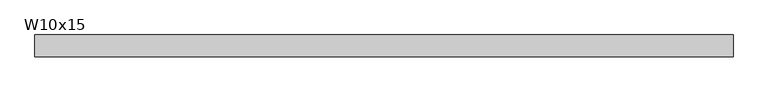
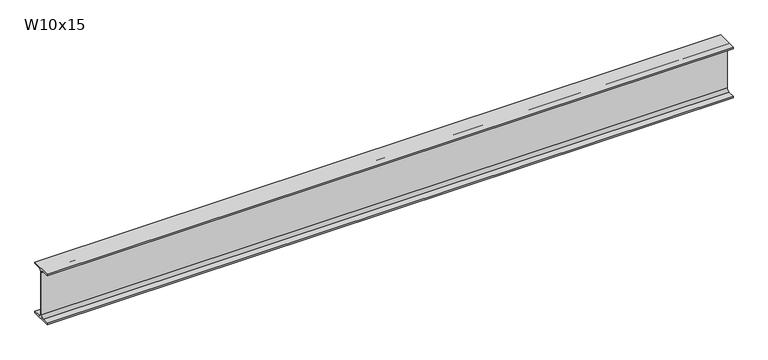
"""IFC4 building model written with IfcOpenShell, lengths in millimetres: beam geometry, RME W-Wide Flange : W10x15."""

import ifcopenshell
import ifcopenshell.guid

model = None  # the IFC model being written
_history = None  # IfcOwnerHistory: only IFC2X3 demands one
_inside = {}  # id of a spatial element -> (the spatial element, [elements in it])
_under = {}  # id of a project, library or spatial element -> (it, [spatial elements below it])
_declared = {}  # id of a project -> (the project, [libraries it declares])
_typed = {}  # id of a type object -> (the type object, [elements of that type])
_made_of = {}  # id of a material, layer set ... -> (it, [elements and type objects made of it])


def new_model(schema):
    """Start an empty IFC model of exactly this schema.

    Asked for "IFC4X3", IfcOpenShell would pick the latest addendum, in which some entities
    have other attributes; the version numbers below select the first issue.
    IFC2X3 requires an IfcOwnerHistory on every rooted entity: one is made here for all.
    """
    global model, _history
    if schema == "IFC4X3":
        model = ifcopenshell.file(schema_version=(4, 3, 0, 0))
    else:
        model = ifcopenshell.file(schema=schema)
    _inside.clear()
    _under.clear()
    _declared.clear()
    _typed.clear()
    _made_of.clear()
    _history = None
    if model.schema == "IFC2X3":
        org = make("IfcOrganization", Name="unknown")
        user = make(
            "IfcPersonAndOrganization",
            ThePerson=make("IfcPerson", FamilyName="unknown"),
            TheOrganization=org,
        )
        app = make(
            "IfcApplication",
            ApplicationDeveloper=org,
            Version="unknown",
            ApplicationFullName="unknown",
            ApplicationIdentifier="unknown",
        )
        _history = make(
            "IfcOwnerHistory",
            OwningUser=user,
            OwningApplication=app,
            ChangeAction="ADDED",
            CreationDate=0,
        )
    return model


def make(cls, **values):
    """One entity of the class cls with the attributes given. An attribute that is None is left unset."""
    return model.create_entity(
        cls, **{name: value for name, value in values.items() if value is not None}
    )


def rooted(cls, **values):
    """An entity with a GlobalId (a new one), such as an element, a storey or a relation."""
    return make(cls, GlobalId=ifcopenshell.guid.new(), OwnerHistory=_history, **values)


def si_unit(unit_type, name, prefix=None):
    """IfcSIUnit, for example si_unit("LENGTHUNIT", "METRE", prefix="MILLI")."""
    return make("IfcSIUnit", UnitType=unit_type, Prefix=prefix, Name=name)


def assignment(units):
    """IfcUnitAssignment: the units of a project."""
    return None if units is None else make("IfcUnitAssignment", Units=units)


def point(xyz):
    """IfcCartesianPoint."""
    return None if xyz is None else make("IfcCartesianPoint", Coordinates=xyz)


def direction(xyz):
    """IfcDirection."""
    return None if xyz is None else make("IfcDirection", DirectionRatios=xyz)


def frame(location, z_axis=None, x_axis=None):
    """IfcAxis2Placement3D, a coordinate frame: its origin and axes. An axis left out is left unset."""
    return make(
        "IfcAxis2Placement3D",
        Location=point(location),
        Axis=direction(z_axis),
        RefDirection=direction(x_axis),
    )


def frame_2d(location, x_axis=None):
    """IfcAxis2Placement2D, a coordinate frame in the plane: its origin and x axis."""
    return make(
        "IfcAxis2Placement2D", Location=point(location), RefDirection=direction(x_axis)
    )


def origin():
    """The frame at (0, 0, 0) with its axes left unset."""
    return frame((0.0, 0.0, 0.0))


def place(relative_to, where):
    """IfcLocalPlacement: puts the frame where relative to a parent placement (None: the world)."""
    return make(
        "IfcLocalPlacement", PlacementRelTo=relative_to, RelativePlacement=where
    )


def context(
    kind, dimensions, precision=None, world=None, true_north=None, identifier=None
):
    """IfcGeometricRepresentationContext, for example the 3D "Model" context."""
    return make(
        "IfcGeometricRepresentationContext",
        ContextIdentifier=identifier,
        ContextType=kind,
        CoordinateSpaceDimension=dimensions,
        Precision=precision,
        WorldCoordinateSystem=world,
        TrueNorth=true_north,
    )


def project(units=None, contexts=None):
    """IfcProject with its units and contexts."""
    return rooted(
        "IfcProject",
        Name="project",
        RepresentationContexts=contexts,
        UnitsInContext=assignment(units),
    )


def spatial(cls, under=None, at=None, **own):
    """A site, building, storey or space (cls), placed at a placement, below another one or the project."""
    s = rooted(cls, ObjectPlacement=at, **own)
    if under is not None:
        _under.setdefault(under.id(), (under, []))[1].append(s)
    return s


def polyline(points):
    """IfcPolyline through the points."""
    return make("IfcPolyline", Points=[point(p) for p in points])


def circle_curve(where, radius):
    """IfcCircle in the frame where."""
    return make("IfcCircle", Position=where, Radius=radius)


def trimmed(basis, trim1, trim2, sense, master):
    """IfcTrimmedCurve: the piece of a basis curve between two trims."""
    return make(
        "IfcTrimmedCurve",
        BasisCurve=basis,
        Trim1=trim1,
        Trim2=trim2,
        SenseAgreement=sense,
        MasterRepresentation=master,
    )


def segment(curve, same_sense, transition):
    """IfcCompositeCurveSegment."""
    return make(
        "IfcCompositeCurveSegment",
        Transition=transition,
        SameSense=same_sense,
        ParentCurve=curve,
    )


def composite_curve(segments, self_intersect=None):
    """IfcCompositeCurve: segments joined end to end."""
    return make("IfcCompositeCurve", Segments=segments, SelfIntersect=self_intersect)


def outline(outer, holes=None, kind="AREA"):
    """IfcArbitraryClosedProfileDef: a profile drawn as a closed curve; with holes, ...WithVoids."""
    if holes is None:
        return make("IfcArbitraryClosedProfileDef", ProfileType=kind, OuterCurve=outer)
    return make(
        "IfcArbitraryProfileDefWithVoids",
        ProfileType=kind,
        OuterCurve=outer,
        InnerCurves=holes,
    )


def extrude(swept, where, along, depth):
    """IfcExtrudedAreaSolid: the profile swept, set in the frame where, extruded along a direction by depth."""
    return make(
        "IfcExtrudedAreaSolid",
        SweptArea=swept,
        Position=where,
        ExtrudedDirection=direction(along),
        Depth=depth,
    )


def shape(context_of_items, identifier, shape_type, items):
    """IfcShapeRepresentation: the items that make up one representation, for example the "Body"."""
    return make(
        "IfcShapeRepresentation",
        ContextOfItems=context_of_items,
        RepresentationIdentifier=identifier,
        RepresentationType=shape_type,
        Items=items,
    )


def source(mapping_origin, context_of_items, identifier, shape_type, items):
    """IfcRepresentationMap: a shape defined once, which mapped items show again and again."""
    return make(
        "IfcRepresentationMap",
        MappingOrigin=mapping_origin,
        MappedRepresentation=shape(context_of_items, identifier, shape_type, items),
    )


def transform(
    local_origin,
    x_axis=None,
    y_axis=None,
    z_axis=None,
    scale=None,
    scale2=None,
    scale3=None,
    uniform=True,
):
    """IfcCartesianTransformationOperator3D, or its non-uniform kind. x_axis, y_axis, z_axis: its Axis1, 2, 3."""
    if uniform:
        return make(
            "IfcCartesianTransformationOperator3D",
            Axis1=direction(x_axis),
            Axis2=direction(y_axis),
            LocalOrigin=point(local_origin),
            Scale=scale,
            Axis3=direction(z_axis),
        )
    return make(
        "IfcCartesianTransformationOperator3DnonUniform",
        Axis1=direction(x_axis),
        Axis2=direction(y_axis),
        LocalOrigin=point(local_origin),
        Scale=scale,
        Axis3=direction(z_axis),
        Scale2=scale2,
        Scale3=scale3,
    )


def mapped(mapping_source, mapping_target):
    """IfcMappedItem: shows the shape of a source again, moved by a transform."""
    return make(
        "IfcMappedItem", MappingSource=mapping_source, MappingTarget=mapping_target
    )


def made_of(thing, what):
    """Note that an element or type object is made of a material, layer set ...; save() writes the relation."""
    if what is not None:
        _made_of.setdefault(what.id(), (what, []))[1].append(thing)
    return thing


def element(
    cls,
    number,
    at=None,
    inside=None,
    cuts=None,
    type_object=None,
    material=None,
    context=None,
    identifier="Body",
    shape_type=None,
    held_by="IfcProductDefinitionShape",
    body=None,
    shapes=None,
    **own,
):
    """One element of the class cls, such as IfcWall. Its Tag is "e" and its number.

    at: its placement. inside: the storey or other place that contains it. cuts: it is an
    opening in that element (IfcRelVoidsElement). A single representation is given by context,
    identifier, shape_type and body (its items); several are given by shapes. held_by: the class
    of the entity that holds the representations. save() writes the other relations.
    """
    e = rooted(cls, Tag="e%d" % number, ObjectPlacement=at, **own)
    if body is not None:
        shapes = [shape(context, identifier, shape_type, body)]
    if shapes is not None:
        e.Representation = make(held_by, Representations=shapes)
    if inside is not None:
        _inside.setdefault(inside.id(), (inside, []))[1].append(e)
    if cuts is not None:
        rooted(
            "IfcRelVoidsElement", RelatingBuildingElement=cuts, RelatedOpeningElement=e
        )
    if type_object is not None:
        _typed.setdefault(type_object.id(), (type_object, []))[1].append(e)
    return made_of(e, material)


def aggregate(whole, parts):
    """IfcRelAggregates: a whole, such as a stair, and the parts it consists of."""
    return rooted("IfcRelAggregates", RelatingObject=whole, RelatedObjects=parts)


def save(model, path):
    """Write the relations noted so far, then the file.

    IfcRelAggregates (storeys below a building ...), IfcRelContainedInSpatialStructure (elements
    in a storey), IfcRelDefinesByType, IfcRelAssociatesMaterial and IfcRelDeclares: one each for
    every whole, place, type object, material and project.
    """
    for whole, parts in _under.values():
        aggregate(whole, parts)
    for where, things in _inside.values():
        rooted(
            "IfcRelContainedInSpatialStructure",
            RelatedElements=things,
            RelatingStructure=where,
        )
    for kind, things in _typed.values():
        rooted("IfcRelDefinesByType", RelatedObjects=things, RelatingType=kind)
    for what, things in _made_of.values():
        rooted("IfcRelAssociatesMaterial", RelatedObjects=things, RelatingMaterial=what)
    for by, libraries in _declared.values():
        rooted("IfcRelDeclares", RelatingContext=by, RelatedDefinitions=libraries)
    model.write(path)


def w10x15_dad78829(model_context):
    return source(origin(), model_context, "Body", "SweptSolid", [
        extrude(outline(composite_curve([segment(polyline([(50.8, -120.142), (50.8, -127.0), (-50.8, -127.0), (-50.8, -120.142), (-16.7005, -120.142)]), True, "CONTINUOUS"), segment(trimmed(circle_curve(frame_2d((-16.7005, -106.3625)), 13.7795), [point((-16.7005, -120.142))], [point((-2.921, -106.3625))], True, "CARTESIAN"), True, "CONTINUOUS"), segment(polyline([(-2.921, -106.3625), (-2.921, 106.3625)]), True, "CONTINUOUS"), segment(trimmed(circle_curve(frame_2d((-16.7005, 106.3625)), 13.7795), [point((-2.921, 106.3625))], [point((-16.7005, 120.142))], True, "CARTESIAN"), True, "CONTINUOUS"), segment(polyline([(-16.7005, 120.142), (-50.8, 120.142), (-50.8, 127.0), (50.8, 127.0), (50.8, 120.142), (16.7005, 120.142)]), True, "CONTINUOUS"), segment(trimmed(circle_curve(frame_2d((16.7005, 106.3625)), 13.7795), [point((16.7005, 120.142))], [point((2.921, 106.3625))], True, "CARTESIAN"), True, "CONTINUOUS"), segment(polyline([(2.921, 106.3625), (2.921, -106.3625)]), True, "CONTINUOUS"), segment(trimmed(circle_curve(frame_2d((16.7005, -106.3625)), 13.7795), [point((2.921, -106.3625))], [point((16.7005, -120.142))], True, "CARTESIAN"), True, "CONTINUOUS"), segment(polyline([(16.7005, -120.142), (50.8, -120.142)]), True, "CONTINUOUS")], self_intersect=False)), frame((-1630.5983978, 0.0, 0.0), z_axis=(1.0, 0.0, 0.0), x_axis=(0.0, 1.0, 0.0)), (0.0, 0.0, 1.0), 3261.1967956),
    ])


if __name__ == "__main__":
    model = new_model("IFC4")
    model_context = context("Model", 3, world=origin())
    ifc_project = project(units=[si_unit("LENGTHUNIT", "METRE", prefix="MILLI")], contexts=[model_context])
    site = spatial("IfcSite", under=ifc_project)
    building = spatial("IfcBuilding", under=site)
    placement = place(None, origin())
    w10x15_shape = w10x15_dad78829(model_context)
    element("IfcBeam", 1, ObjectType="RME W-Wide Flange : W10x15", at=placement, inside=building, context=model_context, shape_type="MappedRepresentation", body=[
        mapped(w10x15_shape, transform((0.0, 0.0, 0.0), x_axis=(1.0, 0.0, 0.0), y_axis=(0.0, 1.0, 0.0), z_axis=(0.0, 0.0, 1.0))),
    ])
    save(model, "model.ifc")

# Revit data of these elements
# Type "RME W-Wide Flange : W10x15"
#   WELD P [instance default] = ""
#   WELD LE [instance default] = ""
#   WELD D [instance default] = ""
#   TOP SECTION SIZE [instance default] = ""
#   TOP SECTION LENGTH [instance default] = ""
#   REMARKS [instance default] = ""
#   REINF TYPE [instance default] = ""
#   Nominal Size = "W24"
#   End Bearing Capacity [instance default] = ""
#   BOT SECTION SIZE [instance default] = ""
#   BOT SECTION LENGTH [instance default] = ""
#   Assembly Code = "B10"
#   W = 15
#   Start Extension Calculation [instance default] = 10' - 0"
#   Start Extension [instance default] = -0' - 0 1/2"
#   End Extension Calculation [instance default] = 10' - 0"
#   End Extension [instance default] = -0' - 0 1/2"
#   Length [instance default] = 5' - 0"
#   bf = 0' - 4"
#   d = 0' - 10"
#   k = 0' - 0 13/16"
#   k2 = 0' - 0.5425"
#   tf = 0' - 0.27"
#   tw = 0' - 0.23"
#   A = 0.030625 SF
#   Structural Material [instance default] = Metal - Steel - ASTM A992
# Element 1 (IfcBeam, "RME W-Wide Flange : W10x15")
#   Length = 10' - 8.39357"
#   Materials on its faces: "Metal - Steel - ASTM A992"
# Materials
#   "Metal - Steel - ASTM A992": class "Metal", colour RGB 255 128 0, transparency 0
